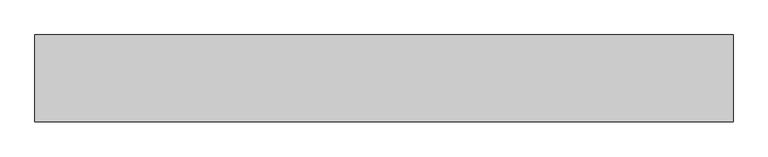
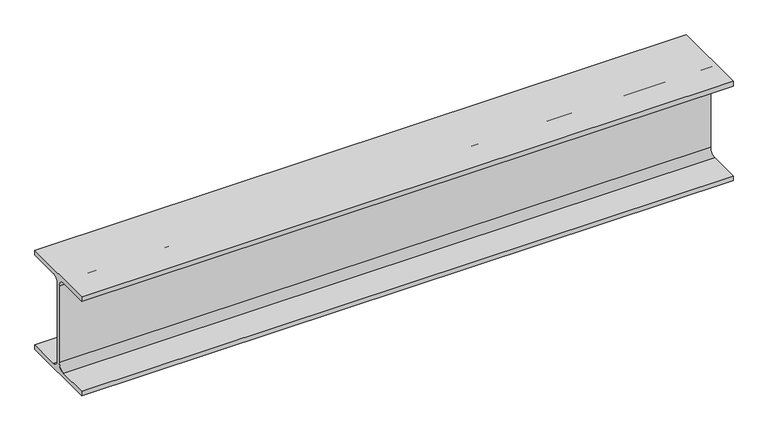
"""IFC4 building model written with IfcOpenShell, lengths in millimetres: beam geometry, 0912_Steel Framing_H-KSD3502 : H_SB_ASB_H-194x150x6x9."""

from ifc_helpers import new_model, si_unit, point, frame, frame_2d, origin, place, context, project, spatial, polyline, circle_curve, trimmed, segment, composite_curve, outline, extrude, source, transform, mapped, element, save


def beam_57c15ec0(model_context):
    return source(origin(), model_context, "Body", "SweptSolid", [
        extrude(outline(composite_curve([segment(polyline([(75.0, -88.0), (75.0, -97.0), (-75.0, -97.0), (-75.0, -88.0), (-16.0, -88.0)]), True, "CONTINUOUS"), segment(trimmed(circle_curve(frame_2d((-16.0, -75.0)), 13.0), [point((-16.0, -88.0))], [point((-3.0, -75.0))], True, "CARTESIAN"), True, "CONTINUOUS"), segment(polyline([(-3.0, -75.0), (-3.0, 75.0)]), True, "CONTINUOUS"), segment(trimmed(circle_curve(frame_2d((-16.0, 75.0)), 13.0), [point((-3.0, 75.0))], [point((-16.0, 88.0))], True, "CARTESIAN"), True, "CONTINUOUS"), segment(polyline([(-16.0, 88.0), (-75.0, 88.0), (-75.0, 97.0), (75.0, 97.0), (75.0, 88.0), (16.0, 88.0)]), True, "CONTINUOUS"), segment(trimmed(circle_curve(frame_2d((16.0, 75.0)), 13.0), [point((16.0, 88.0))], [point((3.0, 75.0))], True, "CARTESIAN"), True, "CONTINUOUS"), segment(polyline([(3.0, 75.0), (3.0, -75.0)]), True, "CONTINUOUS"), segment(trimmed(circle_curve(frame_2d((16.0, -75.0)), 13.0), [point((3.0, -75.0))], [point((16.0, -88.0))], True, "CARTESIAN"), True, "CONTINUOUS"), segment(polyline([(16.0, -88.0), (75.0, -88.0)]), True, "CONTINUOUS")], self_intersect=False)), frame((-601.6366265, 0.0, 0.0), z_axis=(1.0, 0.0, 0.0), x_axis=(0.0, 1.0, 0.0)), (0.0, 0.0, 1.0), 1203.2732531),
    ])


if __name__ == "__main__":
    model = new_model("IFC4")
    model_context = context("Model", 3, world=origin())
    ifc_project = project(units=[si_unit("LENGTHUNIT", "METRE", prefix="MILLI")], contexts=[model_context])
    site = spatial("IfcSite", under=ifc_project)
    building = spatial("IfcBuilding", under=site)
    placement = place(None, origin())
    beam_shape = beam_57c15ec0(model_context)
    element("IfcBeam", 1, ObjectType="0912_Steel Framing_H-KSD3502 : H_SB_ASB_H-194x150x6x9", at=placement, inside=building, context=model_context, shape_type="MappedRepresentation", body=[
        mapped(beam_shape, transform((0.0, 0.0, 0.0), x_axis=(1.0, 0.0, 0.0), y_axis=(0.0, 1.0, 0.0), z_axis=(0.0, 0.0, 1.0))),
    ])
    save(model, "model.ifc")

# Revit data of these elements
# Type "0912_Steel Framing_H-KSD3502 : H_SB_ASB_H-194x150x6x9"
#   H_WM Code_1 = "S01AA002-00001 | Main Steel Structure Fabrication Work | Shelter/Building | Medium Steel - Standard (90KG/M>Weight≥30KG/M) | Material: (   )"
#   H_WM Code_2 = "S03AA028-00001 | Main Steel Structure Erection Work | Shelter/Building | Medium Steel (90KG/M>Weight≥30KG/M) | Material: (   )"
#   H_WM Code_3 = "S01AA010-00001 | Main Steel Structure Fabrication Work | Shelter/Building | Steel Painting/Coating | for Non-Fireproofed Steel Surface, Surface Preparation, Primer, Second & Final Coat | Material: (   )"
#   H_Q'ty Cal Type Tag = "SB-Q2"
#   Width = 15.0 cm
#   Web Thickness = 0.6 cm
#   Web Fillet = 1.3 cm
#   Warping Constant = 43316.0 cm⁶
#   W = 0
#   Torsional Moment of Inertia = 8.622 cm⁴
#   Section Area = 39.01 cm²
#   Plastic Modulus weak axis = 104.0 cm³
#   Plastic Modulus strong axis = 309.0 cm³
#   Perimeter = 0.95 m²/m
#   Nominal Weight = 30.60 kgf/m
#   Moment of Inertia weak axis = 507.00 cm⁴
#   Moment of Inertia strong axis = 2690.00 cm⁴
#   Height = 19.4 cm
#   Flange Thickness = 0.9 cm
#   Elastic Modulus weak axis = 67.6 cm³
#   Elastic Modulus strong axis = 277.0 cm³
#   Centroid Vertical = 9.7 cm
#   Centroid Horizontal = 7.5 cm
#   Ix = 26900000
#   Length [instance default] = 1.5240 m
#   Zx = 309000
#   b = 0.1500 m
#   h = 0.1940 m
#   r = 0.0130 m
#   s = 0.0060 m
#   t = 0.0090 m
#   A = 0.003901 m²
#   Structural Material [instance default] = Steel, 45-345
#   Assembly Code = ""
# Element 1 (IfcBeam, "0912_Steel Framing_H-KSD3502 : H_SB_ASB_H-194x150x6x9")
#   Structural Material = none
# Materials
#   "Steel, 45-345": class "Metal", colour RGB 189 187 185, transparency 0, Description = "Steel 345 MPa", Cost = 0
